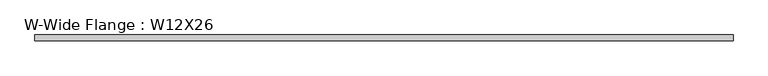
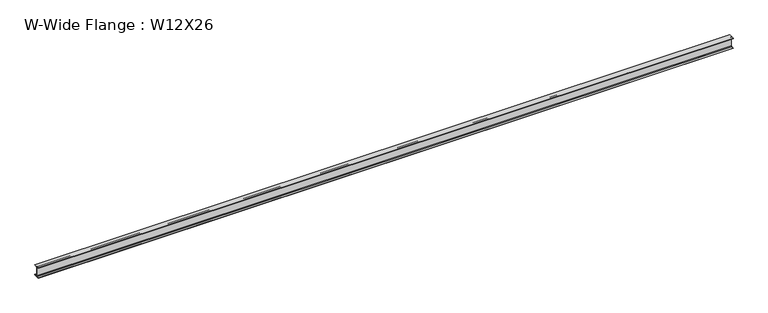
"""IFC4 building model written with IfcOpenShell, lengths in millimetres: beam geometry, W-Wide Flange : W12X26."""

import ifcopenshell
import ifcopenshell.guid

model = None  # the IFC model being written
_history = None  # IfcOwnerHistory: only IFC2X3 demands one
_inside = {}  # id of a spatial element -> (the spatial element, [elements in it])
_under = {}  # id of a project, library or spatial element -> (it, [spatial elements below it])
_declared = {}  # id of a project -> (the project, [libraries it declares])
_typed = {}  # id of a type object -> (the type object, [elements of that type])
_made_of = {}  # id of a material, layer set ... -> (it, [elements and type objects made of it])


def new_model(schema):
    """Start an empty IFC model of exactly this schema.

    Asked for "IFC4X3", IfcOpenShell would pick the latest addendum, in which some entities
    have other attributes; the version numbers below select the first issue.
    IFC2X3 requires an IfcOwnerHistory on every rooted entity: one is made here for all.
    """
    global model, _history
    if schema == "IFC4X3":
        model = ifcopenshell.file(schema_version=(4, 3, 0, 0))
    else:
        model = ifcopenshell.file(schema=schema)
    _inside.clear()
    _under.clear()
    _declared.clear()
    _typed.clear()
    _made_of.clear()
    _history = None
    if model.schema == "IFC2X3":
        org = make("IfcOrganization", Name="unknown")
        user = make(
            "IfcPersonAndOrganization",
            ThePerson=make("IfcPerson", FamilyName="unknown"),
            TheOrganization=org,
        )
        app = make(
            "IfcApplication",
            ApplicationDeveloper=org,
            Version="unknown",
            ApplicationFullName="unknown",
            ApplicationIdentifier="unknown",
        )
        _history = make(
            "IfcOwnerHistory",
            OwningUser=user,
            OwningApplication=app,
            ChangeAction="ADDED",
            CreationDate=0,
        )
    return model


def make(cls, **values):
    """One entity of the class cls with the attributes given. An attribute that is None is left unset."""
    return model.create_entity(
        cls, **{name: value for name, value in values.items() if value is not None}
    )


def rooted(cls, **values):
    """An entity with a GlobalId (a new one), such as an element, a storey or a relation."""
    return make(cls, GlobalId=ifcopenshell.guid.new(), OwnerHistory=_history, **values)


def si_unit(unit_type, name, prefix=None):
    """IfcSIUnit, for example si_unit("LENGTHUNIT", "METRE", prefix="MILLI")."""
    return make("IfcSIUnit", UnitType=unit_type, Prefix=prefix, Name=name)


def assignment(units):
    """IfcUnitAssignment: the units of a project."""
    return None if units is None else make("IfcUnitAssignment", Units=units)


def point(xyz):
    """IfcCartesianPoint."""
    return None if xyz is None else make("IfcCartesianPoint", Coordinates=xyz)


def direction(xyz):
    """IfcDirection."""
    return None if xyz is None else make("IfcDirection", DirectionRatios=xyz)


def frame(location, z_axis=None, x_axis=None):
    """IfcAxis2Placement3D, a coordinate frame: its origin and axes. An axis left out is left unset."""
    return make(
        "IfcAxis2Placement3D",
        Location=point(location),
        Axis=direction(z_axis),
        RefDirection=direction(x_axis),
    )


def frame_2d(location, x_axis=None):
    """IfcAxis2Placement2D, a coordinate frame in the plane: its origin and x axis."""
    return make(
        "IfcAxis2Placement2D", Location=point(location), RefDirection=direction(x_axis)
    )


def origin():
    """The frame at (0, 0, 0) with its axes left unset."""
    return frame((0.0, 0.0, 0.0))


def place(relative_to, where):
    """IfcLocalPlacement: puts the frame where relative to a parent placement (None: the world)."""
    return make(
        "IfcLocalPlacement", PlacementRelTo=relative_to, RelativePlacement=where
    )


def context(
    kind, dimensions, precision=None, world=None, true_north=None, identifier=None
):
    """IfcGeometricRepresentationContext, for example the 3D "Model" context."""
    return make(
        "IfcGeometricRepresentationContext",
        ContextIdentifier=identifier,
        ContextType=kind,
        CoordinateSpaceDimension=dimensions,
        Precision=precision,
        WorldCoordinateSystem=world,
        TrueNorth=true_north,
    )


def project(units=None, contexts=None):
    """IfcProject with its units and contexts."""
    return rooted(
        "IfcProject",
        Name="project",
        RepresentationContexts=contexts,
        UnitsInContext=assignment(units),
    )


def spatial(cls, under=None, at=None, **own):
    """A site, building, storey or space (cls), placed at a placement, below another one or the project."""
    s = rooted(cls, ObjectPlacement=at, **own)
    if under is not None:
        _under.setdefault(under.id(), (under, []))[1].append(s)
    return s


def polyline(points):
    """IfcPolyline through the points."""
    return make("IfcPolyline", Points=[point(p) for p in points])


def circle_curve(where, radius):
    """IfcCircle in the frame where."""
    return make("IfcCircle", Position=where, Radius=radius)


def trimmed(basis, trim1, trim2, sense, master):
    """IfcTrimmedCurve: the piece of a basis curve between two trims."""
    return make(
        "IfcTrimmedCurve",
        BasisCurve=basis,
        Trim1=trim1,
        Trim2=trim2,
        SenseAgreement=sense,
        MasterRepresentation=master,
    )


def segment(curve, same_sense, transition):
    """IfcCompositeCurveSegment."""
    return make(
        "IfcCompositeCurveSegment",
        Transition=transition,
        SameSense=same_sense,
        ParentCurve=curve,
    )


def composite_curve(segments, self_intersect=None):
    """IfcCompositeCurve: segments joined end to end."""
    return make("IfcCompositeCurve", Segments=segments, SelfIntersect=self_intersect)


def outline(outer, holes=None, kind="AREA"):
    """IfcArbitraryClosedProfileDef: a profile drawn as a closed curve; with holes, ...WithVoids."""
    if holes is None:
        return make("IfcArbitraryClosedProfileDef", ProfileType=kind, OuterCurve=outer)
    return make(
        "IfcArbitraryProfileDefWithVoids",
        ProfileType=kind,
        OuterCurve=outer,
        InnerCurves=holes,
    )


def extrude(swept, where, along, depth):
    """IfcExtrudedAreaSolid: the profile swept, set in the frame where, extruded along a direction by depth."""
    return make(
        "IfcExtrudedAreaSolid",
        SweptArea=swept,
        Position=where,
        ExtrudedDirection=direction(along),
        Depth=depth,
    )


def shape(context_of_items, identifier, shape_type, items):
    """IfcShapeRepresentation: the items that make up one representation, for example the "Body"."""
    return make(
        "IfcShapeRepresentation",
        ContextOfItems=context_of_items,
        RepresentationIdentifier=identifier,
        RepresentationType=shape_type,
        Items=items,
    )


def source(mapping_origin, context_of_items, identifier, shape_type, items):
    """IfcRepresentationMap: a shape defined once, which mapped items show again and again."""
    return make(
        "IfcRepresentationMap",
        MappingOrigin=mapping_origin,
        MappedRepresentation=shape(context_of_items, identifier, shape_type, items),
    )


def transform(
    local_origin,
    x_axis=None,
    y_axis=None,
    z_axis=None,
    scale=None,
    scale2=None,
    scale3=None,
    uniform=True,
):
    """IfcCartesianTransformationOperator3D, or its non-uniform kind. x_axis, y_axis, z_axis: its Axis1, 2, 3."""
    if uniform:
        return make(
            "IfcCartesianTransformationOperator3D",
            Axis1=direction(x_axis),
            Axis2=direction(y_axis),
            LocalOrigin=point(local_origin),
            Scale=scale,
            Axis3=direction(z_axis),
        )
    return make(
        "IfcCartesianTransformationOperator3DnonUniform",
        Axis1=direction(x_axis),
        Axis2=direction(y_axis),
        LocalOrigin=point(local_origin),
        Scale=scale,
        Axis3=direction(z_axis),
        Scale2=scale2,
        Scale3=scale3,
    )


def mapped(mapping_source, mapping_target):
    """IfcMappedItem: shows the shape of a source again, moved by a transform."""
    return make(
        "IfcMappedItem", MappingSource=mapping_source, MappingTarget=mapping_target
    )


def made_of(thing, what):
    """Note that an element or type object is made of a material, layer set ...; save() writes the relation."""
    if what is not None:
        _made_of.setdefault(what.id(), (what, []))[1].append(thing)
    return thing


def element(
    cls,
    number,
    at=None,
    inside=None,
    cuts=None,
    type_object=None,
    material=None,
    context=None,
    identifier="Body",
    shape_type=None,
    held_by="IfcProductDefinitionShape",
    body=None,
    shapes=None,
    **own,
):
    """One element of the class cls, such as IfcWall. Its Tag is "e" and its number.

    at: its placement. inside: the storey or other place that contains it. cuts: it is an
    opening in that element (IfcRelVoidsElement). A single representation is given by context,
    identifier, shape_type and body (its items); several are given by shapes. held_by: the class
    of the entity that holds the representations. save() writes the other relations.
    """
    e = rooted(cls, Tag="e%d" % number, ObjectPlacement=at, **own)
    if body is not None:
        shapes = [shape(context, identifier, shape_type, body)]
    if shapes is not None:
        e.Representation = make(held_by, Representations=shapes)
    if inside is not None:
        _inside.setdefault(inside.id(), (inside, []))[1].append(e)
    if cuts is not None:
        rooted(
            "IfcRelVoidsElement", RelatingBuildingElement=cuts, RelatedOpeningElement=e
        )
    if type_object is not None:
        _typed.setdefault(type_object.id(), (type_object, []))[1].append(e)
    return made_of(e, material)


def aggregate(whole, parts):
    """IfcRelAggregates: a whole, such as a stair, and the parts it consists of."""
    return rooted("IfcRelAggregates", RelatingObject=whole, RelatedObjects=parts)


def save(model, path):
    """Write the relations noted so far, then the file.

    IfcRelAggregates (storeys below a building ...), IfcRelContainedInSpatialStructure (elements
    in a storey), IfcRelDefinesByType, IfcRelAssociatesMaterial and IfcRelDeclares: one each for
    every whole, place, type object, material and project.
    """
    for whole, parts in _under.values():
        aggregate(whole, parts)
    for where, things in _inside.values():
        rooted(
            "IfcRelContainedInSpatialStructure",
            RelatedElements=things,
            RelatingStructure=where,
        )
    for kind, things in _typed.values():
        rooted("IfcRelDefinesByType", RelatedObjects=things, RelatingType=kind)
    for what, things in _made_of.values():
        rooted("IfcRelAssociatesMaterial", RelatedObjects=things, RelatingMaterial=what)
    for by, libraries in _declared.values():
        rooted("IfcRelDeclares", RelatingContext=by, RelatedDefinitions=libraries)
    model.write(path)


def w_wide_flange_w12x26_a1de43d1(model_context):
    return source(origin(), model_context, "Body", "SweptSolid", [
        extrude(outline(composite_curve([segment(polyline([(82.4011719, -145.5539063), (82.4011719, -155.178125), (-82.4011719, -155.178125), (-82.4011719, -145.5539063), (-20.2902344, -145.5539063)]), True, "CONTINUOUS"), segment(trimmed(circle_curve(frame_2d((-20.2902344, -128.190625)), 17.3632812), [point((-20.2902344, -145.5539063))], [point((-2.9269531, -128.190625))], True, "CARTESIAN"), True, "CONTINUOUS"), segment(polyline([(-2.9269531, -128.190625), (-2.9269531, 128.190625)]), True, "CONTINUOUS"), segment(trimmed(circle_curve(frame_2d((-20.2902344, 128.190625)), 17.3632812), [point((-2.9269531, 128.190625))], [point((-20.2902344, 145.5539062))], True, "CARTESIAN"), True, "CONTINUOUS"), segment(polyline([(-20.2902344, 145.5539062), (-82.4011719, 145.5539062), (-82.4011719, 155.178125), (82.4011719, 155.178125), (82.4011719, 145.5539062), (20.2902344, 145.5539062)]), True, "CONTINUOUS"), segment(trimmed(circle_curve(frame_2d((20.2902344, 128.190625)), 17.3632812), [point((20.2902344, 145.5539062))], [point((2.9269531, 128.190625))], True, "CARTESIAN"), True, "CONTINUOUS"), segment(polyline([(2.9269531, 128.190625), (2.9269531, -128.190625)]), True, "CONTINUOUS"), segment(trimmed(circle_curve(frame_2d((20.2902344, -128.190625)), 17.3632812), [point((2.9269531, -128.190625))], [point((20.2902344, -145.5539063))], True, "CARTESIAN"), True, "CONTINUOUS"), segment(polyline([(20.2902344, -145.5539063), (82.4011719, -145.5539063)]), True, "CONTINUOUS")], self_intersect=False)), frame((-9944.1, 0.0, 0.0), z_axis=(1.0, 0.0, 0.0), x_axis=(0.0, 1.0, 0.0)), (0.0, 0.0, 1.0), 19888.2),
    ])


if __name__ == "__main__":
    model = new_model("IFC4")
    model_context = context("Model", 3, world=origin())
    ifc_project = project(units=[si_unit("LENGTHUNIT", "METRE", prefix="MILLI")], contexts=[model_context])
    site = spatial("IfcSite", under=ifc_project)
    building = spatial("IfcBuilding", under=site)
    placement = place(None, origin())
    w_wide_flange_w12x26_shape = w_wide_flange_w12x26_a1de43d1(model_context)
    element("IfcBeam", 1, ObjectType="W-Wide Flange : W12X26", at=placement, inside=building, context=model_context, shape_type="MappedRepresentation", body=[
        mapped(w_wide_flange_w12x26_shape, transform((0.0, 0.0, 0.0), x_axis=(1.0, 0.0, 0.0), y_axis=(0.0, 1.0, 0.0), z_axis=(0.0, 0.0, 1.0))),
    ])
    save(model, "model.ifc")

# Revit data of these elements
# Type "W-Wide Flange : W12X26"
#   Assembly Code = "B10"
#   W = 26
#   Length [instance default] = 5' - 0"
#   bf = 0' - 6 125/256"
#   d = 1' - 0 7/32"
#   k = 0' - 1 1/16"
#   k2 = 0' - 0 175/256"
#   tf = 0' - 0 97/256"
#   tw = 0' - 0 59/256"
#   A = 0.053125 SF
#   Structural Material [instance default] = none
# Element 1 (IfcBeam, "W-Wide Flange : W12X26")
#   Structural Material = Dark metal
#   Materials on its faces: "Dark metal"
# Materials
#   "Dark metal": class "Generic", colour RGB 44 29 29, transparency 0, Cost = 0
